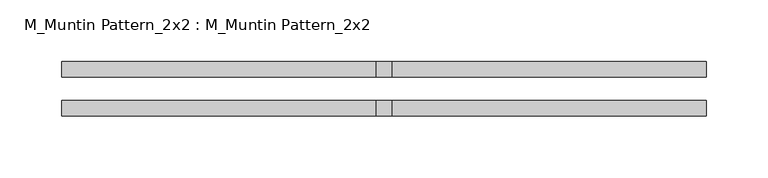
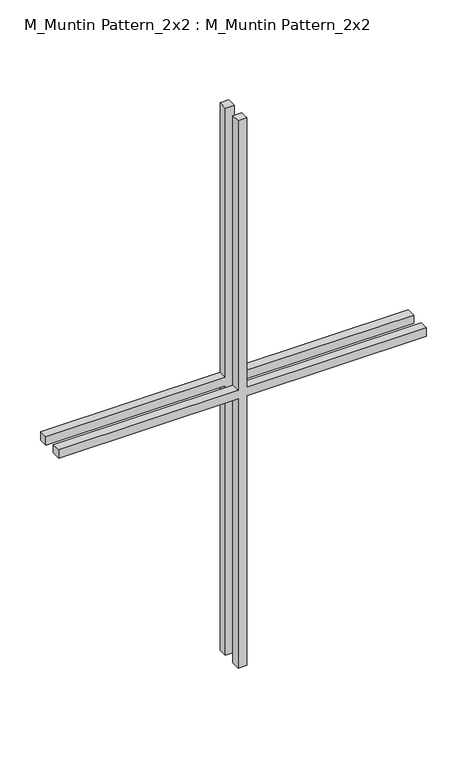
"""IFC4 building model written with IfcOpenShell, lengths in millimetres: proxy geometry, M_Muntin Pattern_2x2 : M_Muntin Pattern_2x2."""

from ifc_helpers import new_model, si_unit, frame, origin, place, context, project, spatial, polyline, outline, extrude, source, transform, mapped, element, save


def m_muntin_pattern_2x2_m_muntin_pattern_2x2_8a7fc2d2(model_context):
    return source(origin(), model_context, "Body", "SweptSolid", [
        extrude(outline(polyline([(418.25, -6.35), (418.25, -261.9), (405.55, -261.9), (405.55, -6.35), (0.0, -6.35), (0.0, 6.35), (405.55, 6.35), (405.55, 261.9), (418.25, 261.9), (418.25, 6.35), (823.8, 6.35), (823.8, -6.35), (418.25, -6.35)])), frame((0.0, -22.225, 0.0), z_axis=(0.0, 1.0, 0.0), x_axis=(0.0, 0.0, 1.0)), (0.0, 0.0, 1.0), 12.7),
        extrude(outline(polyline([(418.25, -6.35), (418.25, -261.9), (405.55, -261.9), (405.55, -6.35), (0.0, -6.35), (0.0, 6.35), (405.55, 6.35), (405.55, 261.9), (418.25, 261.9), (418.25, 6.35), (823.8, 6.35), (823.8, -6.35), (418.25, -6.35)])), frame((0.0, 9.525, 0.0), z_axis=(0.0, 1.0, 0.0), x_axis=(0.0, 0.0, 1.0)), (0.0, 0.0, 1.0), 12.7),
    ])


if __name__ == "__main__":
    model = new_model("IFC4")
    model_context = context("Model", 3, world=origin())
    ifc_project = project(units=[si_unit("LENGTHUNIT", "METRE", prefix="MILLI")], contexts=[model_context])
    site = spatial("IfcSite", under=ifc_project)
    building = spatial("IfcBuilding", under=site)
    placement = place(None, origin())
    m_muntin_pattern_2x2_m_muntin_pattern_2x2_shape = m_muntin_pattern_2x2_m_muntin_pattern_2x2_8a7fc2d2(model_context)
    element("IfcBuildingElementProxy", 1, Name="M_Muntin Pattern_2x2 : M_Muntin Pattern_2x2", ObjectType="M_Muntin Pattern_2x2 : M_Muntin Pattern_2x2", at=placement, inside=building, context=model_context, shape_type="MappedRepresentation", body=[
        mapped(m_muntin_pattern_2x2_m_muntin_pattern_2x2_shape, transform((0.0, 0.0, 0.0), x_axis=(1.0, 0.0, 0.0), y_axis=(0.0, 1.0, 0.0), z_axis=(0.0, 0.0, 1.0))),
    ])
    save(model, "model.ifc")

# Revit data of these elements
# Type "M_Muntin Pattern_2x2 : M_Muntin Pattern_2x2"
#   Width [instance default] = 120 cm
#   Thickness = 1.27 cm
#   Height [instance default] = 120 cm
#   Distance = 1.905 cm
#   Interior Material [instance default] = none
#   Exterior Material [instance default] = none
#   Default Elevation = 0
# Element 1 (IfcBuildingElementProxy, "M_Muntin Pattern_2x2 : M_Muntin Pattern_2x2")
#   Width = 52.38 cm
#   Height = 82.38 cm
#   Interior Material = Wood - Stained
#   Exterior Material = Clad - White
#   Materials on its faces: "Clad - White", "Wood - Stained"
# Materials
#   "Clad - White": class "Wood", colour RGB 245 245 243, transparency 0, Cost = 0
#   "Wood - Stained": class "Wood", colour RGB 173 132 96, transparency 0, Cost = 0
